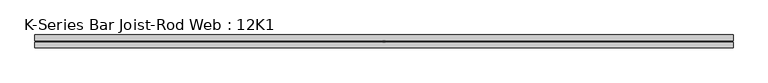
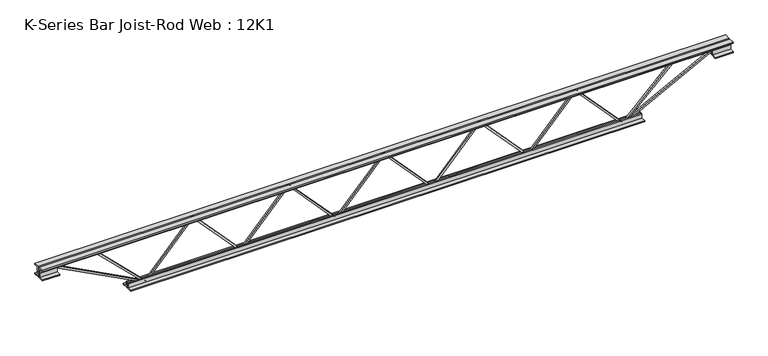
"""IFC4 building model written with IfcOpenShell, lengths in millimetres: beam geometry, K-Series Bar Joist-Rod Web : 12K1."""

import ifcopenshell
import ifcopenshell.guid

model = None  # the IFC model being written
_history = None  # IfcOwnerHistory: only IFC2X3 demands one
_inside = {}  # id of a spatial element -> (the spatial element, [elements in it])
_under = {}  # id of a project, library or spatial element -> (it, [spatial elements below it])
_declared = {}  # id of a project -> (the project, [libraries it declares])
_typed = {}  # id of a type object -> (the type object, [elements of that type])
_made_of = {}  # id of a material, layer set ... -> (it, [elements and type objects made of it])


def new_model(schema):
    """Start an empty IFC model of exactly this schema.

    Asked for "IFC4X3", IfcOpenShell would pick the latest addendum, in which some entities
    have other attributes; the version numbers below select the first issue.
    IFC2X3 requires an IfcOwnerHistory on every rooted entity: one is made here for all.
    """
    global model, _history
    if schema == "IFC4X3":
        model = ifcopenshell.file(schema_version=(4, 3, 0, 0))
    else:
        model = ifcopenshell.file(schema=schema)
    _inside.clear()
    _under.clear()
    _declared.clear()
    _typed.clear()
    _made_of.clear()
    _history = None
    if model.schema == "IFC2X3":
        org = make("IfcOrganization", Name="unknown")
        user = make(
            "IfcPersonAndOrganization",
            ThePerson=make("IfcPerson", FamilyName="unknown"),
            TheOrganization=org,
        )
        app = make(
            "IfcApplication",
            ApplicationDeveloper=org,
            Version="unknown",
            ApplicationFullName="unknown",
            ApplicationIdentifier="unknown",
        )
        _history = make(
            "IfcOwnerHistory",
            OwningUser=user,
            OwningApplication=app,
            ChangeAction="ADDED",
            CreationDate=0,
        )
    return model


def make(cls, **values):
    """One entity of the class cls with the attributes given. An attribute that is None is left unset."""
    return model.create_entity(
        cls, **{name: value for name, value in values.items() if value is not None}
    )


def rooted(cls, **values):
    """An entity with a GlobalId (a new one), such as an element, a storey or a relation."""
    return make(cls, GlobalId=ifcopenshell.guid.new(), OwnerHistory=_history, **values)


def si_unit(unit_type, name, prefix=None):
    """IfcSIUnit, for example si_unit("LENGTHUNIT", "METRE", prefix="MILLI")."""
    return make("IfcSIUnit", UnitType=unit_type, Prefix=prefix, Name=name)


def assignment(units):
    """IfcUnitAssignment: the units of a project."""
    return None if units is None else make("IfcUnitAssignment", Units=units)


def point(xyz):
    """IfcCartesianPoint."""
    return None if xyz is None else make("IfcCartesianPoint", Coordinates=xyz)


def direction(xyz):
    """IfcDirection."""
    return None if xyz is None else make("IfcDirection", DirectionRatios=xyz)


def frame(location, z_axis=None, x_axis=None):
    """IfcAxis2Placement3D, a coordinate frame: its origin and axes. An axis left out is left unset."""
    return make(
        "IfcAxis2Placement3D",
        Location=point(location),
        Axis=direction(z_axis),
        RefDirection=direction(x_axis),
    )


def origin():
    """The frame at (0, 0, 0) with its axes left unset."""
    return frame((0.0, 0.0, 0.0))


def place(relative_to, where):
    """IfcLocalPlacement: puts the frame where relative to a parent placement (None: the world)."""
    return make(
        "IfcLocalPlacement", PlacementRelTo=relative_to, RelativePlacement=where
    )


def context(
    kind, dimensions, precision=None, world=None, true_north=None, identifier=None
):
    """IfcGeometricRepresentationContext, for example the 3D "Model" context."""
    return make(
        "IfcGeometricRepresentationContext",
        ContextIdentifier=identifier,
        ContextType=kind,
        CoordinateSpaceDimension=dimensions,
        Precision=precision,
        WorldCoordinateSystem=world,
        TrueNorth=true_north,
    )


def project(units=None, contexts=None):
    """IfcProject with its units and contexts."""
    return rooted(
        "IfcProject",
        Name="project",
        RepresentationContexts=contexts,
        UnitsInContext=assignment(units),
    )


def spatial(cls, under=None, at=None, **own):
    """A site, building, storey or space (cls), placed at a placement, below another one or the project."""
    s = rooted(cls, ObjectPlacement=at, **own)
    if under is not None:
        _under.setdefault(under.id(), (under, []))[1].append(s)
    return s


def polyline(points):
    """IfcPolyline through the points."""
    return make("IfcPolyline", Points=[point(p) for p in points])


def outline(outer, holes=None, kind="AREA"):
    """IfcArbitraryClosedProfileDef: a profile drawn as a closed curve; with holes, ...WithVoids."""
    if holes is None:
        return make("IfcArbitraryClosedProfileDef", ProfileType=kind, OuterCurve=outer)
    return make(
        "IfcArbitraryProfileDefWithVoids",
        ProfileType=kind,
        OuterCurve=outer,
        InnerCurves=holes,
    )


def extrude(swept, where, along, depth):
    """IfcExtrudedAreaSolid: the profile swept, set in the frame where, extruded along a direction by depth."""
    return make(
        "IfcExtrudedAreaSolid",
        SweptArea=swept,
        Position=where,
        ExtrudedDirection=direction(along),
        Depth=depth,
    )


def shape(context_of_items, identifier, shape_type, items):
    """IfcShapeRepresentation: the items that make up one representation, for example the "Body"."""
    return make(
        "IfcShapeRepresentation",
        ContextOfItems=context_of_items,
        RepresentationIdentifier=identifier,
        RepresentationType=shape_type,
        Items=items,
    )


def source(mapping_origin, context_of_items, identifier, shape_type, items):
    """IfcRepresentationMap: a shape defined once, which mapped items show again and again."""
    return make(
        "IfcRepresentationMap",
        MappingOrigin=mapping_origin,
        MappedRepresentation=shape(context_of_items, identifier, shape_type, items),
    )


def transform(
    local_origin,
    x_axis=None,
    y_axis=None,
    z_axis=None,
    scale=None,
    scale2=None,
    scale3=None,
    uniform=True,
):
    """IfcCartesianTransformationOperator3D, or its non-uniform kind. x_axis, y_axis, z_axis: its Axis1, 2, 3."""
    if uniform:
        return make(
            "IfcCartesianTransformationOperator3D",
            Axis1=direction(x_axis),
            Axis2=direction(y_axis),
            LocalOrigin=point(local_origin),
            Scale=scale,
            Axis3=direction(z_axis),
        )
    return make(
        "IfcCartesianTransformationOperator3DnonUniform",
        Axis1=direction(x_axis),
        Axis2=direction(y_axis),
        LocalOrigin=point(local_origin),
        Scale=scale,
        Axis3=direction(z_axis),
        Scale2=scale2,
        Scale3=scale3,
    )


def mapped(mapping_source, mapping_target):
    """IfcMappedItem: shows the shape of a source again, moved by a transform."""
    return make(
        "IfcMappedItem", MappingSource=mapping_source, MappingTarget=mapping_target
    )


def made_of(thing, what):
    """Note that an element or type object is made of a material, layer set ...; save() writes the relation."""
    if what is not None:
        _made_of.setdefault(what.id(), (what, []))[1].append(thing)
    return thing


def element(
    cls,
    number,
    at=None,
    inside=None,
    cuts=None,
    type_object=None,
    material=None,
    context=None,
    identifier="Body",
    shape_type=None,
    held_by="IfcProductDefinitionShape",
    body=None,
    shapes=None,
    **own,
):
    """One element of the class cls, such as IfcWall. Its Tag is "e" and its number.

    at: its placement. inside: the storey or other place that contains it. cuts: it is an
    opening in that element (IfcRelVoidsElement). A single representation is given by context,
    identifier, shape_type and body (its items); several are given by shapes. held_by: the class
    of the entity that holds the representations. save() writes the other relations.
    """
    e = rooted(cls, Tag="e%d" % number, ObjectPlacement=at, **own)
    if body is not None:
        shapes = [shape(context, identifier, shape_type, body)]
    if shapes is not None:
        e.Representation = make(held_by, Representations=shapes)
    if inside is not None:
        _inside.setdefault(inside.id(), (inside, []))[1].append(e)
    if cuts is not None:
        rooted(
            "IfcRelVoidsElement", RelatingBuildingElement=cuts, RelatedOpeningElement=e
        )
    if type_object is not None:
        _typed.setdefault(type_object.id(), (type_object, []))[1].append(e)
    return made_of(e, material)


def aggregate(whole, parts):
    """IfcRelAggregates: a whole, such as a stair, and the parts it consists of."""
    return rooted("IfcRelAggregates", RelatingObject=whole, RelatedObjects=parts)


def save(model, path):
    """Write the relations noted so far, then the file.

    IfcRelAggregates (storeys below a building ...), IfcRelContainedInSpatialStructure (elements
    in a storey), IfcRelDefinesByType, IfcRelAssociatesMaterial and IfcRelDeclares: one each for
    every whole, place, type object, material and project.
    """
    for whole, parts in _under.values():
        aggregate(whole, parts)
    for where, things in _inside.values():
        rooted(
            "IfcRelContainedInSpatialStructure",
            RelatedElements=things,
            RelatingStructure=where,
        )
    for kind, things in _typed.values():
        rooted("IfcRelDefinesByType", RelatedObjects=things, RelatingType=kind)
    for what, things in _made_of.values():
        rooted("IfcRelAssociatesMaterial", RelatedObjects=things, RelatingMaterial=what)
    for by, libraries in _declared.values():
        rooted("IfcRelDeclares", RelatingContext=by, RelatedDefinitions=libraries)
    model.write(path)


def k_series_bar_joist_rod_web_12k1_d719edf7(model_context):
    return source(origin(), model_context, "Body", "SweptSolid", [
        extrude(outline(polyline([(-141.2875, 274.32), (-150.8125, 274.32), (-150.8125, 279.5889133), (141.2875, 547.5589133), (141.2875, 549.7210867), (-150.8125, 817.6910867), (-150.8125, 822.96), (-141.2875, 822.96), (-141.2875, 821.8789133), (150.8125, 553.9089133), (150.8125, 543.3710867), (-141.2875, 275.4010867), (-141.2875, 274.32)])), frame((0.0, -4.7625, 0.0), z_axis=(0.0, 1.0, 0.0), x_axis=(0.0, 0.0, 1.0)), (0.0, 0.0, 1.0), 9.525),
        extrude(outline(polyline([(-141.2875, -274.32), (-150.8125, -274.32), (-150.8125, -269.0510867), (141.2875, -1.0810867), (141.2875, 1.0810867), (-150.8125, 269.0510867), (-150.8125, 274.32), (-141.2875, 274.32), (-141.2875, 273.2389133), (150.8125, 5.2689133), (150.8125, -5.2689133), (-141.2875, -273.2389133), (-141.2875, -274.32)])), frame((0.0, -4.7625, 0.0), z_axis=(0.0, 1.0, 0.0), x_axis=(0.0, 0.0, 1.0)), (0.0, 0.0, 1.0), 9.525),
        extrude(outline(polyline([(-141.2875, -822.96), (-150.8125, -822.96), (-150.8125, -817.6910867), (141.2875, -549.7210867), (141.2875, -547.5589133), (-150.8125, -279.5889133), (-150.8125, -274.32), (-141.2875, -274.32), (-141.2875, -275.4010867), (150.8125, -543.3710867), (150.8125, -553.9089133), (-141.2875, -821.8789133), (-141.2875, -822.96)])), frame((0.0, -4.7625, 0.0), z_axis=(0.0, 1.0, 0.0), x_axis=(0.0, 0.0, 1.0)), (0.0, 0.0, 1.0), 9.525),
        extrude(outline(polyline([(-141.2875, 822.96), (-150.8125, 822.96), (-150.8125, 828.2289133), (141.2875, 1096.1989133), (141.2875, 1098.3610867), (-150.8125, 1366.3310867), (-150.8125, 1371.6), (-141.2875, 1371.6), (-141.2875, 1370.5189133), (150.8125, 1102.5489133), (150.8125, 1092.0110867), (-141.2875, 824.0410867), (-141.2875, 822.96)])), frame((0.0, -4.7625, 0.0), z_axis=(0.0, 1.0, 0.0), x_axis=(0.0, 0.0, 1.0)), (0.0, 0.0, 1.0), 9.525),
        extrude(outline(polyline([(-141.2875, -1371.6), (-150.8125, -1371.6), (-150.8125, -1366.3310867), (141.2875, -1098.3610867), (141.2875, -1096.1989133), (-150.8125, -828.2289133), (-150.8125, -822.96), (-141.2875, -822.96), (-141.2875, -824.0410867), (150.8125, -1092.0110867), (150.8125, -1102.5489133), (-141.2875, -1370.5189133), (-141.2875, -1371.6)])), frame((0.0, -4.7625, 0.0), z_axis=(0.0, 1.0, 0.0), x_axis=(0.0, 0.0, 1.0)), (0.0, 0.0, 1.0), 9.525),
        extrude(outline(polyline([(4.7625, 152.4), (36.5125, 152.4), (36.5125, 146.05), (11.1125, 146.05), (11.1125, 120.65), (4.7625, 120.65), (4.7625, 152.4)])), frame((-1981.2, 0.0, 0.0), z_axis=(1.0, 0.0, 0.0), x_axis=(0.0, 1.0, 0.0)), (0.0, 0.0, 1.0), 3962.4),
        extrude(outline(polyline([(-4.7625, 152.4), (-4.7625, 120.65), (-11.1125, 120.65), (-11.1125, 146.05), (-36.5125, 146.05), (-36.5125, 152.4), (-4.7625, 152.4)])), frame((-1981.2, 0.0, 0.0), z_axis=(1.0, 0.0, 0.0), x_axis=(0.0, 1.0, 0.0)), (0.0, 0.0, 1.0), 3962.4),
        extrude(outline(polyline([(-4.7625, 88.9), (-36.5125, 88.9), (-36.5125, 95.25), (-11.1125, 95.25), (-11.1125, 120.65), (-4.7625, 120.65), (-4.7625, 88.9)])), frame((-1981.2, 0.0, 0.0), z_axis=(1.0, 0.0, 0.0), x_axis=(0.0, 1.0, 0.0)), (0.0, 0.0, 1.0), 101.6),
        extrude(outline(polyline([(36.5125, 88.9), (4.7625, 88.9), (4.7625, 120.65), (11.1125, 120.65), (11.1125, 95.25), (36.5125, 95.25), (36.5125, 88.9)])), frame((-1981.2, 0.0, 0.0), z_axis=(1.0, 0.0, 0.0), x_axis=(0.0, 1.0, 0.0)), (0.0, 0.0, 1.0), 101.6),
        extrude(outline(polyline([(4.7625, 88.9), (4.7625, 120.65), (11.1125, 120.65), (11.1125, 95.25), (36.5125, 95.25), (36.5125, 88.9), (4.7625, 88.9)])), frame((1879.6, 0.0, 0.0), z_axis=(1.0, 0.0, 0.0), x_axis=(0.0, 1.0, 0.0)), (0.0, 0.0, 1.0), 101.6),
        extrude(outline(polyline([(-4.7625, 88.9), (-36.5125, 88.9), (-36.5125, 95.25), (-11.1125, 95.25), (-11.1125, 120.65), (-4.7625, 120.65), (-4.7625, 88.9)])), frame((1879.6, 0.0, 0.0), z_axis=(1.0, 0.0, 0.0), x_axis=(0.0, 1.0, 0.0)), (0.0, 0.0, 1.0), 101.6),
        extrude(outline(polyline([(4.7625, -152.4), (4.7625, -120.65), (11.1125, -120.65), (11.1125, -146.05), (36.5125, -146.05), (36.5125, -152.4), (4.7625, -152.4)])), frame((-1473.2, 0.0, 0.0), z_axis=(1.0, 0.0, 0.0), x_axis=(0.0, 1.0, 0.0)), (0.0, 0.0, 1.0), 2946.4),
        extrude(outline(polyline([(-4.7625, -152.4), (-36.5125, -152.4), (-36.5125, -146.05), (-11.1125, -146.05), (-11.1125, -120.65), (-4.7625, -120.65), (-4.7625, -152.4)])), frame((-1473.2, 0.0, 0.0), z_axis=(1.0, 0.0, 0.0), x_axis=(0.0, 1.0, 0.0)), (0.0, 0.0, 1.0), 2946.4),
        extrude(outline(polyline([(0.0, -9.525), (0.0, 0.0), (573.7533355, 0.0), (573.7533355, -9.525), (0.0, -9.525)])), frame((-1881.8137714, 4.7625, 116.4332925), z_axis=(0.46483389898951427, 0.0, 0.8853979028381568), x_axis=(0.8853979028381568, 0.0, -0.46483389898951427)), (0.0, 0.0, 1.0), 9.525),
        extrude(outline(polyline([(0.0, -9.525), (0.0, 0.0), (382.5968536, 0.0), (382.5968536, -9.525), (0.0, -9.525)])), frame((-1649.2398358, 4.7625, 117.2353117), z_axis=(0.6970783932914373, 0.0, 0.7169949188147908), x_axis=(0.7169949188147908, 0.0, -0.6970783932914373)), (0.0, 0.0, 1.0), 9.525),
        extrude(outline(polyline([(0.0, -9.525), (0.0, 0.0), (573.7533355, 0.0), (573.7533355, -9.525), (0.0, -9.525)])), frame((1881.8137714, -4.7625, 116.4332925), z_axis=(-0.4648338989894953, 0.0, 0.8853979028381667), x_axis=(-0.8853979028381667, 0.0, -0.4648338989894953)), (0.0, 0.0, 1.0), 9.525),
        extrude(outline(polyline([(0.0, -9.525), (0.0, 0.0), (382.5968536, 0.0), (382.5968536, -9.525), (0.0, -9.525)])), frame((1649.2398358, -4.7625, 117.2353117), z_axis=(-0.6970783932914311, 0.0, 0.7169949188147967), x_axis=(-0.7169949188147967, 0.0, -0.6970783932914311)), (0.0, 0.0, 1.0), 9.525),
    ])


if __name__ == "__main__":
    model = new_model("IFC4")
    model_context = context("Model", 3, world=origin())
    ifc_project = project(units=[si_unit("LENGTHUNIT", "METRE", prefix="MILLI")], contexts=[model_context])
    site = spatial("IfcSite", under=ifc_project)
    building = spatial("IfcBuilding", under=site)
    placement = place(None, origin())
    k_series_bar_joist_rod_web_12k1_shape = k_series_bar_joist_rod_web_12k1_d719edf7(model_context)
    element("IfcBeam", 1, ObjectType="K-Series Bar Joist-Rod Web : 12K1", at=placement, inside=building, context=model_context, shape_type="MappedRepresentation", body=[
        mapped(k_series_bar_joist_rod_web_12k1_shape, transform((0.0, 0.0, 0.0), x_axis=(1.0, 0.0, 0.0), y_axis=(0.0, 1.0, 0.0), z_axis=(0.0, 0.0, 1.0))),
    ])
    save(model, "model.ifc")

# Revit data of these elements
# Type "K-Series Bar Joist-Rod Web : 12K1"
#   Assembly Code = "B1010350"
#   Wt = 5
#   Web Thickness = 0' - 0 3/8"
#   Start Offset [instance default] = 0' - 0"
#   Start Extension [instance default] = 0' - 0"
#   Seat Length = 0' - 4"
#   Seat Depth = 0' - 2 1/2"
#   PanelArrayLength [instance default] = 20' - 0"
#   Panel [instance default] = 2' - 0"
#   End Offset [instance default] = 0' - 0"
#   End Extension [instance default] = 0' - 0"
#   End Panel = 2' - 0"
#   Cord Leg = 0' - 1 1/4"
#   Chord Thickness = 0' - 0 1/4"
#   Length [instance default] = 24' - 0"
#   Depth = 1' - 0"
#   PanelArrayNum [instance default] = 10
#   Structural Material = none
# Element 1 (IfcBeam, "K-Series Bar Joist-Rod Web : 12K1")
#   PanelArrayLength = 9' - 0"
#   Panel = 1' - 9.6"
#   PanelArrayNum = 5
